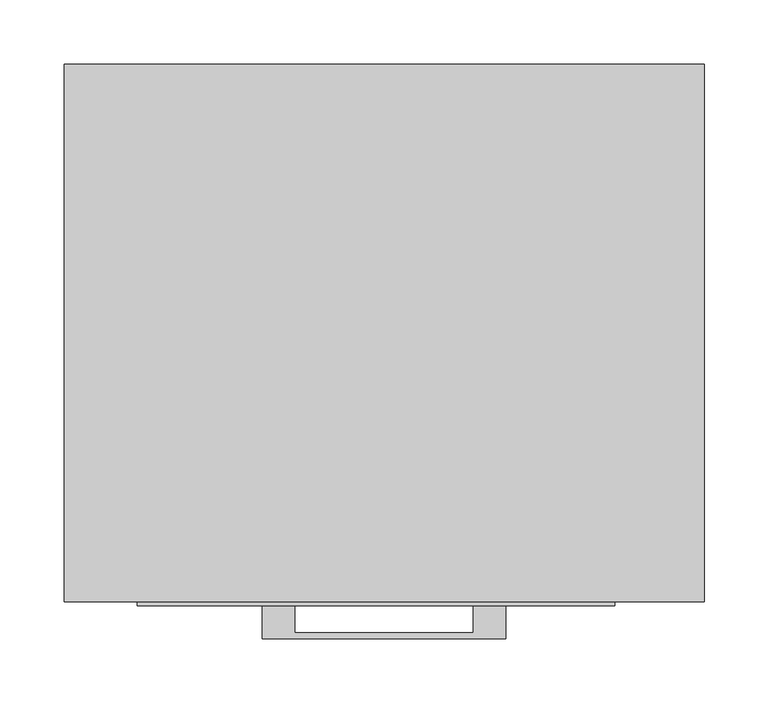
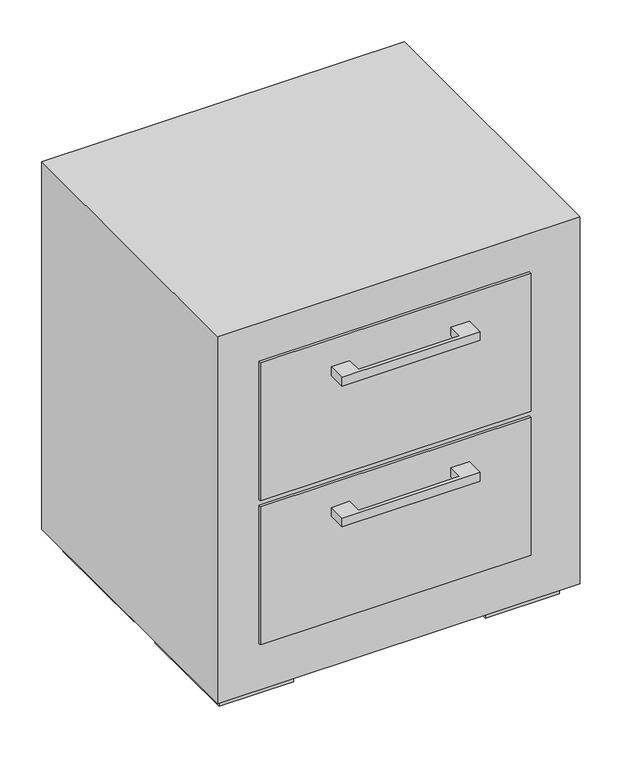
"""IFC4 building model written with IfcOpenShell, lengths in millimetres: furniture geometry, Criado mudo : Criado mudo."""

from ifc_helpers import new_model, si_unit, frame, origin, origin_with_axes, place, context, project, spatial, polyline, outline, extrude, source, transform, mapped, element, save


def furniture_79364497(model_context):
    return source(origin(), model_context, "Body", "SweptSolid", [
        extrude(outline(polyline([(-135.8627073, -12.7), (-135.8627073, -182.0169665), (-238.2627073, -182.0169665), (-238.2627073, -12.7), (-135.8627073, -12.7)])), origin_with_axes(), (0.0, 0.0, 1.0), 14.9168536),
        extrude(outline(polyline([(234.8846936, -12.7), (234.8846936, -182.0169665), (125.1934917, -182.0169665), (125.1934917, -12.7), (234.8846936, -12.7)])), origin_with_axes(), (0.0, 0.0, 1.0), 14.9168536),
        extrude(outline(polyline([(-135.8627073, -232.8169665), (-135.8627073, -385.2169665), (-238.2627073, -385.2169665), (-238.2627073, -232.8169665), (-135.8627073, -232.8169665)])), origin_with_axes(), (0.0, 0.0, 1.0), 14.9168536),
        extrude(outline(polyline([(231.5448501, -232.8169665), (231.5448501, -385.2169665), (129.2372927, -385.2169665), (129.2372927, -232.8169665), (231.5448501, -232.8169665)])), origin_with_axes(), (0.0, 0.0, 1.0), 14.9168536),
        extrude(outline(polyline([(182.5, -401.0919665), (-190.5, -401.0919665), (-190.5, -397.9169665), (182.5, -397.9169665), (182.5, -401.0919665)])), frame((0.0, 0.0, 292.55), z_axis=(0.0, 0.0, 1.0), x_axis=(1.0, 0.0, 0.0)), (0.0, 0.0, 1.0), 201.6125),
        extrude(outline(polyline([(-92.9, -427.0311125), (-92.9, -401.6311125), (-67.5, -401.6311125), (-67.5, -422.2686125), (72.2, -422.2686125), (72.2, -401.6311125), (97.6, -401.6311125), (97.6, -427.0311125), (-92.9, -427.0311125)])), frame((0.0, 0.0, 236.3666599), z_axis=(0.0, 0.0, 1.0), x_axis=(1.0, 0.0, 0.0)), (0.0, 0.0, 1.0), 12.7),
        extrude(outline(polyline([(-92.9, -427.0311125), (-92.9, -401.6311125), (-67.5, -401.6311125), (-67.5, -422.2686125), (72.2, -422.2686125), (72.2, -401.6311125), (97.6, -401.6311125), (97.6, -427.0311125), (-92.9, -427.0311125)])), frame((0.0, 0.0, 441.3666599), z_axis=(0.0, 0.0, 1.0), x_axis=(1.0, 0.0, 0.0)), (0.0, 0.0, 1.0), 12.7),
        extrude(outline(polyline([(182.5, -401.0919665), (-190.5, -401.0919665), (-190.5, -397.9169665), (182.5, -397.9169665), (182.5, -401.0919665)])), frame((0.0, 0.0, 82.55), z_axis=(0.0, 0.0, 1.0), x_axis=(1.0, 0.0, 0.0)), (0.0, 0.0, 1.0), 201.6125),
        extrude(outline(polyline([(252.35, 22.0830335), (252.35, -397.9169665), (-247.65, -397.9169665), (-247.65, 22.0830335), (252.35, 22.0830335)])), frame((0.0, 0.0, 14.9168536), z_axis=(0.0, 0.0, 1.0), x_axis=(1.0, 0.0, 0.0)), (0.0, 0.0, 1.0), 535.0831464),
    ])


if __name__ == "__main__":
    model = new_model("IFC4")
    model_context = context("Model", 3, world=origin())
    ifc_project = project(units=[si_unit("LENGTHUNIT", "METRE", prefix="MILLI")], contexts=[model_context])
    site = spatial("IfcSite", under=ifc_project)
    building = spatial("IfcBuilding", under=site)
    placement = place(None, origin())
    furniture_shape = furniture_79364497(model_context)
    element("IfcFurniture", 1, ObjectType="Criado mudo : Criado mudo", at=placement, inside=building, context=model_context, shape_type="MappedRepresentation", body=[
        mapped(furniture_shape, transform((0.0, 0.0, 0.0), x_axis=(1.0, 0.0, 0.0), y_axis=(0.0, 1.0, 0.0), z_axis=(0.0, 0.0, 1.0))),
    ])
    save(model, "model.ifc")

# Revit data of these elements
# Type "Criado mudo : Criado mudo"
#   Profundidade = 0.42 m
#   Largura = 0.5 m
#   Altura = 0.55 m
#   Material = wood brown
#   Puxador = Handle
# Element 1 (IfcFurniture, "Criado mudo : Criado mudo")
#   Materials on its faces: "wood brown", "Handle"
# Materials
#   "wood brown": class "Wood", colour RGB 80 39 12, transparency 0, Cost = 0
#   "Handle": class "Não atribuído", colour RGB 247 247 247, transparency 0, Cost = 0
